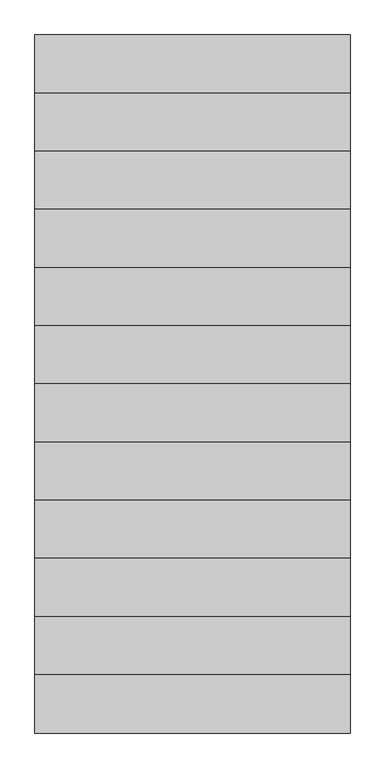
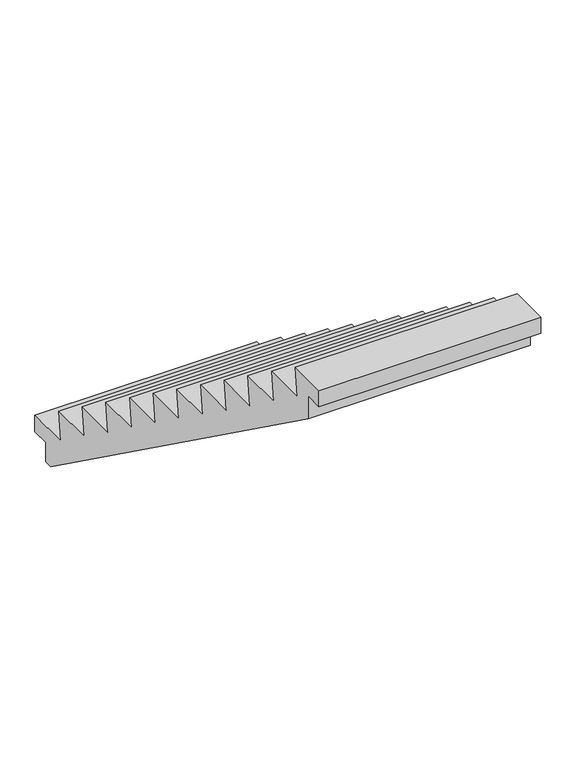
"""IFC4 building model written with IfcOpenShell, lengths in millimetres: proxy geometry, NLRS_24_GM_LB_rechte steektrap prefab-AV_gen_rsf : prefab trap_gen__aant=11 b=1200 a=220 o=172.7 zonder bomen."""

from ifc_helpers import new_model, si_unit, frame, origin, place, context, project, spatial, polyline, outline, extrude, source, transform, mapped, element, save


def generic_models_c6ebb296(model_context):
    return source(origin(), model_context, "Body", "SweptSolid", [
        extrude(outline(polyline([(-2400.0, 1900.0), (-2420.0, 1727.2727273), (-2160.0, 1727.2727273), (-2180.0, 1554.5454545), (-1920.0, 1554.5454545), (-1940.0, 1381.8181818), (-1680.0, 1381.8181818), (-1700.0, 1209.0909091), (-1440.0, 1209.0909091), (-1460.0, 1036.3636364), (-1200.0, 1036.3636364), (-1220.0, 863.6363636), (-960.0, 863.6363636), (-980.0, 690.9090909), (-720.0, 690.9090909), (-740.0, 518.1818182), (-480.0, 518.1818182), (-500.0, 345.4545455), (-240.0, 345.4545455), (-260.0, 172.7272727), (0.0, 172.7272727), (-20.0, 0.0), (240.0, 0.0), (240.0, -100.0), (130.0, -100.0), (130.0, -220.0), (80.254966, -220.0), (-2530.0, 1658.5925892), (-2530.0, 1800.0), (-2640.0, 1800.0), (-2640.0, 1900.0), (-2400.0, 1900.0)])), frame((-650.0, 0.0, 0.0), z_axis=(1.0, 0.0, 0.0), x_axis=(0.0, 1.0, 0.0)), (0.0, 0.0, 1.0), 1300.0),
    ])


if __name__ == "__main__":
    model = new_model("IFC4")
    model_context = context("Model", 3, world=origin())
    ifc_project = project(units=[si_unit("LENGTHUNIT", "METRE", prefix="MILLI")], contexts=[model_context])
    site = spatial("IfcSite", under=ifc_project)
    building = spatial("IfcBuilding", under=site)
    placement = place(None, origin())
    generic_models_shape = generic_models_c6ebb296(model_context)
    element("IfcBuildingElementProxy", 1, Name="NLRS_24_GM_LB_rechte steektrap prefab-AV_gen_rsf : prefab trap_gen__aant=11 b=1200 a=220 o=172.7 zonder bomen", ObjectType="NLRS_24_GM_LB_rechte steektrap prefab-AV_gen_rsf : prefab trap_gen__aant=11 b=1200 a=220 o=172.7 zonder bomen", at=placement, inside=building, context=model_context, shape_type="MappedRepresentation", body=[
        mapped(generic_models_shape, transform((0.0, 0.0, 0.0), x_axis=(1.0, 0.0, 0.0), y_axis=(0.0, 1.0, 0.0), z_axis=(0.0, 0.0, 1.0))),
    ])
    save(model, "model.ifc")

# Revit data of these elements
# Type "NLRS_24_GM_LB_rechte steektrap prefab-AV_gen_rsf : prefab trap_gen__aant=11 b=1200 a=220 o=172.7 zonder bomen"
#   Export Type to IFC As = "IfcStair"
#   Type IfcGUID = "2CEqVLPNH8KRN7ghwV3Z03"
#   Type Comments = " "
#   Model = " "
#   Manufacturer = " "
#   Keynote = " "
#   Description = "rechte steektrap prefab\r\naant=11 b=1200 a=220 o=181,8\r\nzonder bomen"
#   Assembly Code = "24.11"
#   Aantrede onder = 240 mm
#   Width = 1300 mm
#   Wel diepte = 20 mm
#   Trapboom breedte = 0 mm
#   Thickness = 120 mm
#   Optrede onderste trede = 220 mm
#   NLRS_C_lengte = 2400 mm
#   Length = 2880 mm
#   Hoogte oplegnok onder = 100 mm
#   Hoogte oplegnok boven = 100 mm
#   Height = 1900 mm
#   Breedte oplegnok boven = 110 mm
#   BottomCalc = 0 mm
#   Actual Tread Depth = 240 mm
#   Actual Riser Height = 172.727 mm
#   Actual Number of Tread = 10
#   Actual Number of Risers = 11
#   Aantrede boven = 240 mm
#   Aantal treden max dertig = 11
#   Trapboom = no
#   Oplegnok onder = yes
#   NLRS_C_materiaal = NLRS_f2_beton prefab_gen_rsf
#   Default Elevation = 0
# Element 1 (IfcBuildingElementProxy, "NLRS_24_GM_LB_rechte steektrap prefab-AV_gen_rsf : prefab trap_gen__aant=11 b=1200 a=220 o=172.7 zonder bomen")
#   Materials on its faces: "NLRS_f2_beton prefab_gen_rsf"
# Materials
#   "NLRS_f2_beton prefab_gen_rsf": class "F - Niet gebakken kunststeen", colour RGB 129 133 118, transparency 0, Keynote = "f2", Manufacturer = "Revit Standards Foundation", URL = "www.revitstandards.org", Description = "beton prefab", Cost = 0
